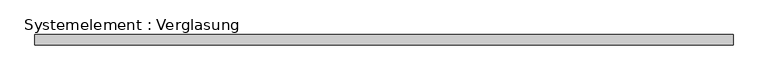
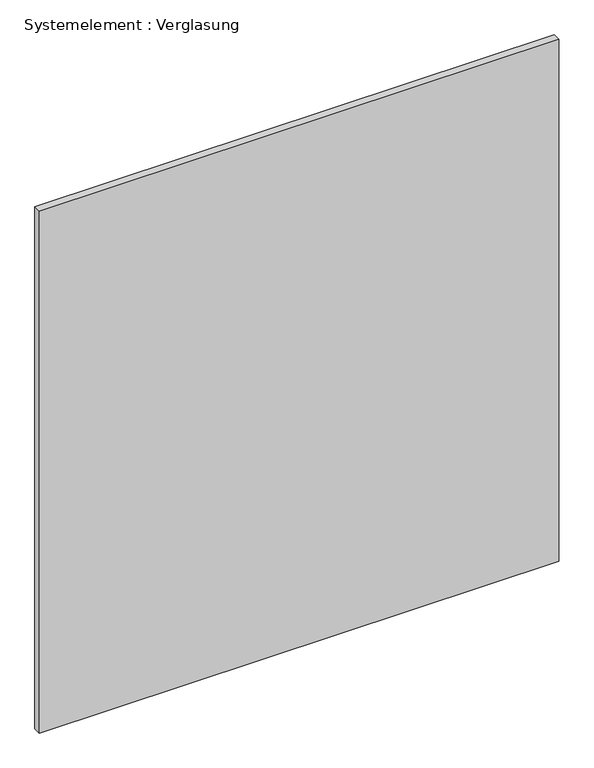
"""IFC4 building model written with IfcOpenShell, lengths in millimetres: plate geometry, Systemelement : Verglasung."""

from ifc_helpers import new_model, si_unit, origin, origin_with_axes, place, context, project, spatial, polyline, outline, extrude, source, transform, mapped, element, save


def systemelement_verglasung_8ef497e6(model_context):
    return source(origin(), model_context, "Body", "SweptSolid", [
        extrude(outline(polyline([(1025.0000002, -15.0), (-1025.0000002, -15.0), (-1025.0000002, 15.0), (1025.0000002, 15.0), (1025.0000002, -15.0)])), origin_with_axes(), (0.0, 0.0, 1.0), 2177.088502),
    ])


if __name__ == "__main__":
    model = new_model("IFC4")
    model_context = context("Model", 3, world=origin())
    ifc_project = project(units=[si_unit("LENGTHUNIT", "METRE", prefix="MILLI")], contexts=[model_context])
    site = spatial("IfcSite", under=ifc_project)
    building = spatial("IfcBuilding", under=site)
    placement = place(None, origin())
    systemelement_verglasung_shape = systemelement_verglasung_8ef497e6(model_context)
    element("IfcPlate", 1, ObjectType="Systemelement : Verglasung", at=placement, inside=building, context=model_context, shape_type="MappedRepresentation", body=[
        mapped(systemelement_verglasung_shape, transform((0.0, 0.0, 0.0), x_axis=(1.0, 0.0, 0.0), y_axis=(0.0, 1.0, 0.0), z_axis=(0.0, 0.0, 1.0))),
    ])
    save(model, "model.ifc")

# Revit data of these elements
# Type "Systemelement : Verglasung"
#   Construction Type Id = "GSP4R"
#   Analytic Construction = "1/8 Zoll Pilkington-Verglasung einfach"
#   Visual Light Transmittance = 0.9
#   Solar Heat Gain Coefficient = 0.86
#   Heat Transfer Coefficient (U) = 6.7069 W/(m²·K)
# Element 1 (IfcPlate, "Systemelement : Verglasung")
#   Materials on its faces: "Glas"
# Materials
#   "Glas": class "Glas", colour RGB 0 0 255, transparency 0.75, Comments = "Render-Darstellung nicht aktualisiert ", Cost = 0
